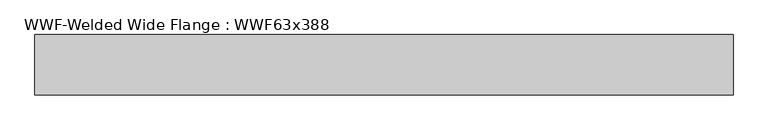
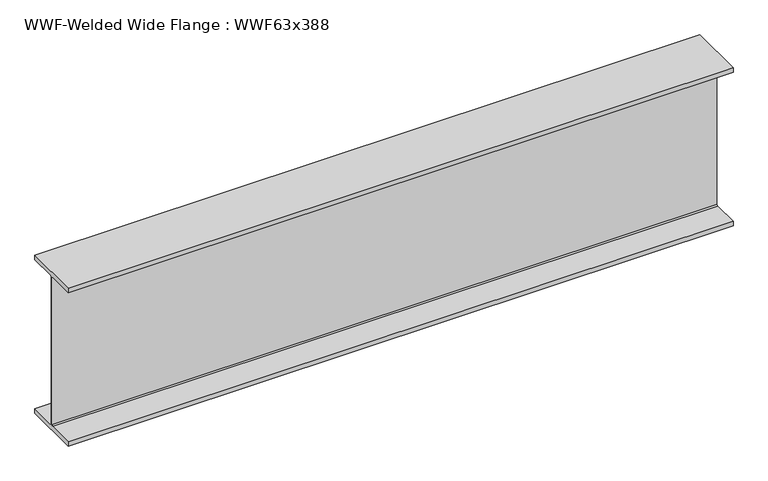
"""IFC4 building model written with IfcOpenShell, lengths in millimetres: beam geometry, WWF-Welded Wide Flange : WWF63x388."""

from ifc_helpers import new_model, si_unit, frame, origin, place, context, project, spatial, polyline, outline, extrude, source, transform, mapped, element, save


def wwf_welded_wide_flange_wwf63x388_0f283b3f(model_context):
    return source(origin(), model_context, "Body", "SweptSolid", [
        extrude(outline(polyline([(274.955, -755.015), (274.955, -799.973), (-274.955, -799.973), (-274.955, -755.015), (-19.05, -755.015), (-8.001, -743.966), (-8.001, 743.966), (-19.05, 755.015), (-274.955, 755.015), (-274.955, 799.973), (274.955, 799.973), (274.955, 755.015), (19.05, 755.015), (8.001, 743.966), (8.001, -743.966), (19.05, -755.015), (274.955, -755.015)])), frame((-3184.5801954, 0.0, 0.0), z_axis=(1.0, 0.0, 0.0), x_axis=(0.0, 1.0, 0.0)), (0.0, 0.0, 1.0), 6369.1344444),
    ])


if __name__ == "__main__":
    model = new_model("IFC4")
    model_context = context("Model", 3, world=origin())
    ifc_project = project(units=[si_unit("LENGTHUNIT", "METRE", prefix="MILLI")], contexts=[model_context])
    site = spatial("IfcSite", under=ifc_project)
    building = spatial("IfcBuilding", under=site)
    placement = place(None, origin())
    wwf_welded_wide_flange_wwf63x388_shape = wwf_welded_wide_flange_wwf63x388_0f283b3f(model_context)
    element("IfcBeam", 1, ObjectType="WWF-Welded Wide Flange : WWF63x388", at=placement, inside=building, context=model_context, shape_type="MappedRepresentation", body=[
        mapped(wwf_welded_wide_flange_wwf63x388_shape, transform((0.0, 0.0, 0.0), x_axis=(1.0, 0.0, 0.0), y_axis=(0.0, 1.0, 0.0), z_axis=(0.0, 0.0, 1.0))),
    ])
    save(model, "model.ifc")

# Revit data of these elements
# Type "WWF-Welded Wide Flange : WWF63x388"
#   Assembly Code = "B10"
#   Nominal d = "12"
#   W = 388
#   Length [instance default] = 1524 mm
#   bf = 549.91 mm
#   d = 1599.946 mm
#   k = 19.05 mm
#   tf = 44.958 mm
#   tw = 16.002 mm
#   A = 0.0735482 m²
#   Structural Material [instance default] = Steel ASTM A572
# Element 1 (IfcBeam, "WWF-Welded Wide Flange : WWF63x388")
#   Structural Material = Metal - Steel 43-275
#   Materials on its faces: "Metal - Steel 43-275"
# Materials
#   "Steel ASTM A572": class "Metal", colour RGB 247 247 247, transparency 0, Description = "Structural steel, high strength low alloy, ASTM - A572 - 50", Cost = 0
#   "Metal - Steel 43-275": class "Metal", colour RGB 247 247 247, transparency 0, Cost = 0
